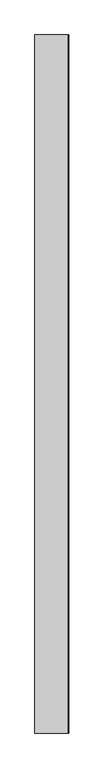
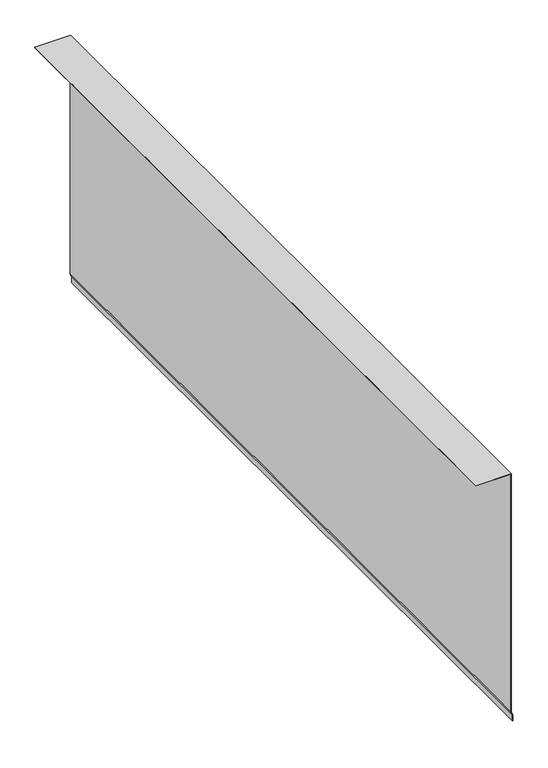
"""IFC4 building model written with IfcOpenShell, lengths in millimetres: proxy geometry, Membrane057 4599 : Membrane057 4599."""

import ifcopenshell
import ifcopenshell.guid

model = None  # the IFC model being written
_history = None  # IfcOwnerHistory: only IFC2X3 demands one
_inside = {}  # id of a spatial element -> (the spatial element, [elements in it])
_under = {}  # id of a project, library or spatial element -> (it, [spatial elements below it])
_declared = {}  # id of a project -> (the project, [libraries it declares])
_typed = {}  # id of a type object -> (the type object, [elements of that type])
_made_of = {}  # id of a material, layer set ... -> (it, [elements and type objects made of it])


def new_model(schema):
    """Start an empty IFC model of exactly this schema.

    Asked for "IFC4X3", IfcOpenShell would pick the latest addendum, in which some entities
    have other attributes; the version numbers below select the first issue.
    IFC2X3 requires an IfcOwnerHistory on every rooted entity: one is made here for all.
    """
    global model, _history
    if schema == "IFC4X3":
        model = ifcopenshell.file(schema_version=(4, 3, 0, 0))
    else:
        model = ifcopenshell.file(schema=schema)
    _inside.clear()
    _under.clear()
    _declared.clear()
    _typed.clear()
    _made_of.clear()
    _history = None
    if model.schema == "IFC2X3":
        org = make("IfcOrganization", Name="unknown")
        user = make(
            "IfcPersonAndOrganization",
            ThePerson=make("IfcPerson", FamilyName="unknown"),
            TheOrganization=org,
        )
        app = make(
            "IfcApplication",
            ApplicationDeveloper=org,
            Version="unknown",
            ApplicationFullName="unknown",
            ApplicationIdentifier="unknown",
        )
        _history = make(
            "IfcOwnerHistory",
            OwningUser=user,
            OwningApplication=app,
            ChangeAction="ADDED",
            CreationDate=0,
        )
    return model


def make(cls, **values):
    """One entity of the class cls with the attributes given. An attribute that is None is left unset."""
    return model.create_entity(
        cls, **{name: value for name, value in values.items() if value is not None}
    )


def rooted(cls, **values):
    """An entity with a GlobalId (a new one), such as an element, a storey or a relation."""
    return make(cls, GlobalId=ifcopenshell.guid.new(), OwnerHistory=_history, **values)


def si_unit(unit_type, name, prefix=None):
    """IfcSIUnit, for example si_unit("LENGTHUNIT", "METRE", prefix="MILLI")."""
    return make("IfcSIUnit", UnitType=unit_type, Prefix=prefix, Name=name)


def assignment(units):
    """IfcUnitAssignment: the units of a project."""
    return None if units is None else make("IfcUnitAssignment", Units=units)


def point(xyz):
    """IfcCartesianPoint."""
    return None if xyz is None else make("IfcCartesianPoint", Coordinates=xyz)


def direction(xyz):
    """IfcDirection."""
    return None if xyz is None else make("IfcDirection", DirectionRatios=xyz)


def frame(location, z_axis=None, x_axis=None):
    """IfcAxis2Placement3D, a coordinate frame: its origin and axes. An axis left out is left unset."""
    return make(
        "IfcAxis2Placement3D",
        Location=point(location),
        Axis=direction(z_axis),
        RefDirection=direction(x_axis),
    )


def origin():
    """The frame at (0, 0, 0) with its axes left unset."""
    return frame((0.0, 0.0, 0.0))


def place(relative_to, where):
    """IfcLocalPlacement: puts the frame where relative to a parent placement (None: the world)."""
    return make(
        "IfcLocalPlacement", PlacementRelTo=relative_to, RelativePlacement=where
    )


def context(
    kind, dimensions, precision=None, world=None, true_north=None, identifier=None
):
    """IfcGeometricRepresentationContext, for example the 3D "Model" context."""
    return make(
        "IfcGeometricRepresentationContext",
        ContextIdentifier=identifier,
        ContextType=kind,
        CoordinateSpaceDimension=dimensions,
        Precision=precision,
        WorldCoordinateSystem=world,
        TrueNorth=true_north,
    )


def project(units=None, contexts=None):
    """IfcProject with its units and contexts."""
    return rooted(
        "IfcProject",
        Name="project",
        RepresentationContexts=contexts,
        UnitsInContext=assignment(units),
    )


def spatial(cls, under=None, at=None, **own):
    """A site, building, storey or space (cls), placed at a placement, below another one or the project."""
    s = rooted(cls, ObjectPlacement=at, **own)
    if under is not None:
        _under.setdefault(under.id(), (under, []))[1].append(s)
    return s


def polyline(points):
    """IfcPolyline through the points."""
    return make("IfcPolyline", Points=[point(p) for p in points])


def outline(outer, holes=None, kind="AREA"):
    """IfcArbitraryClosedProfileDef: a profile drawn as a closed curve; with holes, ...WithVoids."""
    if holes is None:
        return make("IfcArbitraryClosedProfileDef", ProfileType=kind, OuterCurve=outer)
    return make(
        "IfcArbitraryProfileDefWithVoids",
        ProfileType=kind,
        OuterCurve=outer,
        InnerCurves=holes,
    )


def extrude(swept, where, along, depth):
    """IfcExtrudedAreaSolid: the profile swept, set in the frame where, extruded along a direction by depth."""
    return make(
        "IfcExtrudedAreaSolid",
        SweptArea=swept,
        Position=where,
        ExtrudedDirection=direction(along),
        Depth=depth,
    )


def shape(context_of_items, identifier, shape_type, items):
    """IfcShapeRepresentation: the items that make up one representation, for example the "Body"."""
    return make(
        "IfcShapeRepresentation",
        ContextOfItems=context_of_items,
        RepresentationIdentifier=identifier,
        RepresentationType=shape_type,
        Items=items,
    )


def source(mapping_origin, context_of_items, identifier, shape_type, items):
    """IfcRepresentationMap: a shape defined once, which mapped items show again and again."""
    return make(
        "IfcRepresentationMap",
        MappingOrigin=mapping_origin,
        MappedRepresentation=shape(context_of_items, identifier, shape_type, items),
    )


def transform(
    local_origin,
    x_axis=None,
    y_axis=None,
    z_axis=None,
    scale=None,
    scale2=None,
    scale3=None,
    uniform=True,
):
    """IfcCartesianTransformationOperator3D, or its non-uniform kind. x_axis, y_axis, z_axis: its Axis1, 2, 3."""
    if uniform:
        return make(
            "IfcCartesianTransformationOperator3D",
            Axis1=direction(x_axis),
            Axis2=direction(y_axis),
            LocalOrigin=point(local_origin),
            Scale=scale,
            Axis3=direction(z_axis),
        )
    return make(
        "IfcCartesianTransformationOperator3DnonUniform",
        Axis1=direction(x_axis),
        Axis2=direction(y_axis),
        LocalOrigin=point(local_origin),
        Scale=scale,
        Axis3=direction(z_axis),
        Scale2=scale2,
        Scale3=scale3,
    )


def mapped(mapping_source, mapping_target):
    """IfcMappedItem: shows the shape of a source again, moved by a transform."""
    return make(
        "IfcMappedItem", MappingSource=mapping_source, MappingTarget=mapping_target
    )


def made_of(thing, what):
    """Note that an element or type object is made of a material, layer set ...; save() writes the relation."""
    if what is not None:
        _made_of.setdefault(what.id(), (what, []))[1].append(thing)
    return thing


def element(
    cls,
    number,
    at=None,
    inside=None,
    cuts=None,
    type_object=None,
    material=None,
    context=None,
    identifier="Body",
    shape_type=None,
    held_by="IfcProductDefinitionShape",
    body=None,
    shapes=None,
    **own,
):
    """One element of the class cls, such as IfcWall. Its Tag is "e" and its number.

    at: its placement. inside: the storey or other place that contains it. cuts: it is an
    opening in that element (IfcRelVoidsElement). A single representation is given by context,
    identifier, shape_type and body (its items); several are given by shapes. held_by: the class
    of the entity that holds the representations. save() writes the other relations.
    """
    e = rooted(cls, Tag="e%d" % number, ObjectPlacement=at, **own)
    if body is not None:
        shapes = [shape(context, identifier, shape_type, body)]
    if shapes is not None:
        e.Representation = make(held_by, Representations=shapes)
    if inside is not None:
        _inside.setdefault(inside.id(), (inside, []))[1].append(e)
    if cuts is not None:
        rooted(
            "IfcRelVoidsElement", RelatingBuildingElement=cuts, RelatedOpeningElement=e
        )
    if type_object is not None:
        _typed.setdefault(type_object.id(), (type_object, []))[1].append(e)
    return made_of(e, material)


def aggregate(whole, parts):
    """IfcRelAggregates: a whole, such as a stair, and the parts it consists of."""
    return rooted("IfcRelAggregates", RelatingObject=whole, RelatedObjects=parts)


def save(model, path):
    """Write the relations noted so far, then the file.

    IfcRelAggregates (storeys below a building ...), IfcRelContainedInSpatialStructure (elements
    in a storey), IfcRelDefinesByType, IfcRelAssociatesMaterial and IfcRelDeclares: one each for
    every whole, place, type object, material and project.
    """
    for whole, parts in _under.values():
        aggregate(whole, parts)
    for where, things in _inside.values():
        rooted(
            "IfcRelContainedInSpatialStructure",
            RelatedElements=things,
            RelatingStructure=where,
        )
    for kind, things in _typed.values():
        rooted("IfcRelDefinesByType", RelatedObjects=things, RelatingType=kind)
    for what, things in _made_of.values():
        rooted("IfcRelAssociatesMaterial", RelatedObjects=things, RelatingMaterial=what)
    for by, libraries in _declared.values():
        rooted("IfcRelDeclares", RelatingContext=by, RelatedDefinitions=libraries)
    model.write(path)


def generic_models_312b7eb8(model_context):
    return source(origin(), model_context, "Body", "SweptSolid", [
        extrude(outline(polyline([(40237.828125, -4494.3379668), (40236.828125, -4494.3379668), (40236.828125, -4401.7658618), (39579.3230707, -4401.7658618), (39568.0978055, -4397.6801994), (39552.6918208, -4397.6801994), (39552.6918208, -4396.6801994), (39568.2741325, -4396.6801994), (39579.4993977, -4400.7658618), (40237.828125, -4400.7658618), (40237.828125, -4494.3379668)])), frame((0.0, -1065.3406572, 0.0), z_axis=(0.0, 1.0, 0.0), x_axis=(0.0, 0.0, 1.0)), (0.0, 0.0, 1.0), 2000.0),
    ])


if __name__ == "__main__":
    model = new_model("IFC4")
    model_context = context("Model", 3, world=origin())
    ifc_project = project(units=[si_unit("LENGTHUNIT", "METRE", prefix="MILLI")], contexts=[model_context])
    site = spatial("IfcSite", under=ifc_project)
    building = spatial("IfcBuilding", under=site)
    placement = place(None, origin())
    generic_models_shape = generic_models_312b7eb8(model_context)
    element("IfcBuildingElementProxy", 1, Name="Membrane057 4599 : Membrane057 4599", ObjectType="Membrane057 4599 : Membrane057 4599", at=placement, inside=building, context=model_context, shape_type="MappedRepresentation", body=[
        mapped(generic_models_shape, transform((0.0, 0.0, 0.0), x_axis=(1.0, 0.0, 0.0), y_axis=(0.0, 1.0, 0.0), z_axis=(0.0, 0.0, 1.0))),
    ])
    save(model, "model.ifc")

# Revit data of these elements
# Type "Membrane057 4599 : Membrane057 4599"
#   NameOverride = "Membrane057"
# Element 1 (IfcBuildingElementProxy, "Membrane057 4599 : Membrane057 4599")
#   Materials on its faces: "2 LAYERS NO. 30 ASTM D226 ASPHALT SATURATED ORGANIC FELT"
# Materials
#   "2 LAYERS NO. 30 ASTM D226 ASPHALT SATURATED ORGANIC FELT": class "Unassigned", colour RGB 46 171 0, transparency 0
